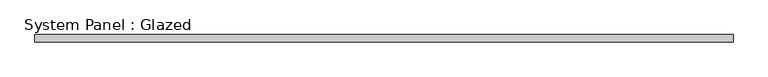
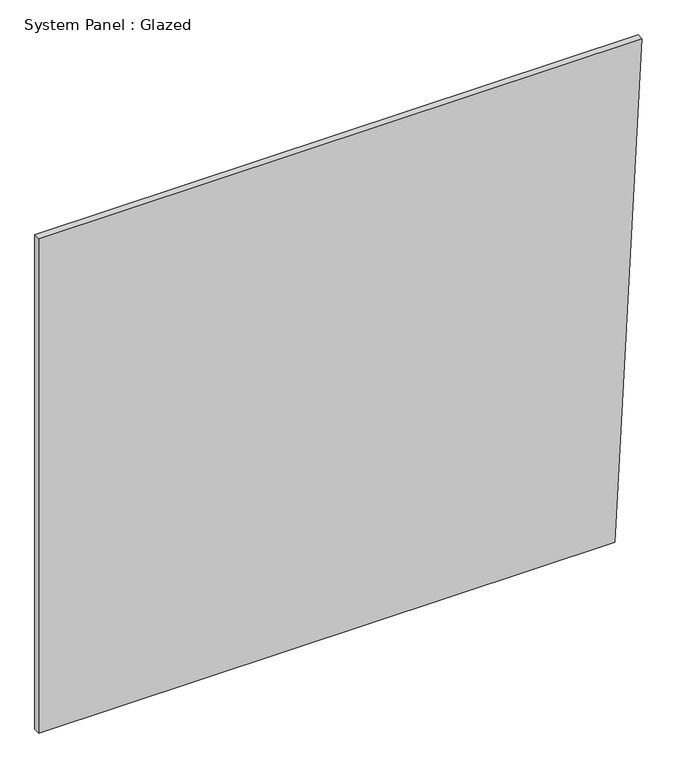
"""IFC4 building model written with IfcOpenShell, lengths in millimetres: plate geometry, System Panel : Glazed."""

import ifcopenshell
import ifcopenshell.guid

model = None  # the IFC model being written
_history = None  # IfcOwnerHistory: only IFC2X3 demands one
_inside = {}  # id of a spatial element -> (the spatial element, [elements in it])
_under = {}  # id of a project, library or spatial element -> (it, [spatial elements below it])
_declared = {}  # id of a project -> (the project, [libraries it declares])
_typed = {}  # id of a type object -> (the type object, [elements of that type])
_made_of = {}  # id of a material, layer set ... -> (it, [elements and type objects made of it])


def new_model(schema):
    """Start an empty IFC model of exactly this schema.

    Asked for "IFC4X3", IfcOpenShell would pick the latest addendum, in which some entities
    have other attributes; the version numbers below select the first issue.
    IFC2X3 requires an IfcOwnerHistory on every rooted entity: one is made here for all.
    """
    global model, _history
    if schema == "IFC4X3":
        model = ifcopenshell.file(schema_version=(4, 3, 0, 0))
    else:
        model = ifcopenshell.file(schema=schema)
    _inside.clear()
    _under.clear()
    _declared.clear()
    _typed.clear()
    _made_of.clear()
    _history = None
    if model.schema == "IFC2X3":
        org = make("IfcOrganization", Name="unknown")
        user = make(
            "IfcPersonAndOrganization",
            ThePerson=make("IfcPerson", FamilyName="unknown"),
            TheOrganization=org,
        )
        app = make(
            "IfcApplication",
            ApplicationDeveloper=org,
            Version="unknown",
            ApplicationFullName="unknown",
            ApplicationIdentifier="unknown",
        )
        _history = make(
            "IfcOwnerHistory",
            OwningUser=user,
            OwningApplication=app,
            ChangeAction="ADDED",
            CreationDate=0,
        )
    return model


def make(cls, **values):
    """One entity of the class cls with the attributes given. An attribute that is None is left unset."""
    return model.create_entity(
        cls, **{name: value for name, value in values.items() if value is not None}
    )


def rooted(cls, **values):
    """An entity with a GlobalId (a new one), such as an element, a storey or a relation."""
    return make(cls, GlobalId=ifcopenshell.guid.new(), OwnerHistory=_history, **values)


def si_unit(unit_type, name, prefix=None):
    """IfcSIUnit, for example si_unit("LENGTHUNIT", "METRE", prefix="MILLI")."""
    return make("IfcSIUnit", UnitType=unit_type, Prefix=prefix, Name=name)


def assignment(units):
    """IfcUnitAssignment: the units of a project."""
    return None if units is None else make("IfcUnitAssignment", Units=units)


def point(xyz):
    """IfcCartesianPoint."""
    return None if xyz is None else make("IfcCartesianPoint", Coordinates=xyz)


def direction(xyz):
    """IfcDirection."""
    return None if xyz is None else make("IfcDirection", DirectionRatios=xyz)


def frame(location, z_axis=None, x_axis=None):
    """IfcAxis2Placement3D, a coordinate frame: its origin and axes. An axis left out is left unset."""
    return make(
        "IfcAxis2Placement3D",
        Location=point(location),
        Axis=direction(z_axis),
        RefDirection=direction(x_axis),
    )


def origin():
    """The frame at (0, 0, 0) with its axes left unset."""
    return frame((0.0, 0.0, 0.0))


def place(relative_to, where):
    """IfcLocalPlacement: puts the frame where relative to a parent placement (None: the world)."""
    return make(
        "IfcLocalPlacement", PlacementRelTo=relative_to, RelativePlacement=where
    )


def context(
    kind, dimensions, precision=None, world=None, true_north=None, identifier=None
):
    """IfcGeometricRepresentationContext, for example the 3D "Model" context."""
    return make(
        "IfcGeometricRepresentationContext",
        ContextIdentifier=identifier,
        ContextType=kind,
        CoordinateSpaceDimension=dimensions,
        Precision=precision,
        WorldCoordinateSystem=world,
        TrueNorth=true_north,
    )


def project(units=None, contexts=None):
    """IfcProject with its units and contexts."""
    return rooted(
        "IfcProject",
        Name="project",
        RepresentationContexts=contexts,
        UnitsInContext=assignment(units),
    )


def spatial(cls, under=None, at=None, **own):
    """A site, building, storey or space (cls), placed at a placement, below another one or the project."""
    s = rooted(cls, ObjectPlacement=at, **own)
    if under is not None:
        _under.setdefault(under.id(), (under, []))[1].append(s)
    return s


def polyline(points):
    """IfcPolyline through the points."""
    return make("IfcPolyline", Points=[point(p) for p in points])


def outline(outer, holes=None, kind="AREA"):
    """IfcArbitraryClosedProfileDef: a profile drawn as a closed curve; with holes, ...WithVoids."""
    if holes is None:
        return make("IfcArbitraryClosedProfileDef", ProfileType=kind, OuterCurve=outer)
    return make(
        "IfcArbitraryProfileDefWithVoids",
        ProfileType=kind,
        OuterCurve=outer,
        InnerCurves=holes,
    )


def extrude(swept, where, along, depth):
    """IfcExtrudedAreaSolid: the profile swept, set in the frame where, extruded along a direction by depth."""
    return make(
        "IfcExtrudedAreaSolid",
        SweptArea=swept,
        Position=where,
        ExtrudedDirection=direction(along),
        Depth=depth,
    )


def shape(context_of_items, identifier, shape_type, items):
    """IfcShapeRepresentation: the items that make up one representation, for example the "Body"."""
    return make(
        "IfcShapeRepresentation",
        ContextOfItems=context_of_items,
        RepresentationIdentifier=identifier,
        RepresentationType=shape_type,
        Items=items,
    )


def source(mapping_origin, context_of_items, identifier, shape_type, items):
    """IfcRepresentationMap: a shape defined once, which mapped items show again and again."""
    return make(
        "IfcRepresentationMap",
        MappingOrigin=mapping_origin,
        MappedRepresentation=shape(context_of_items, identifier, shape_type, items),
    )


def transform(
    local_origin,
    x_axis=None,
    y_axis=None,
    z_axis=None,
    scale=None,
    scale2=None,
    scale3=None,
    uniform=True,
):
    """IfcCartesianTransformationOperator3D, or its non-uniform kind. x_axis, y_axis, z_axis: its Axis1, 2, 3."""
    if uniform:
        return make(
            "IfcCartesianTransformationOperator3D",
            Axis1=direction(x_axis),
            Axis2=direction(y_axis),
            LocalOrigin=point(local_origin),
            Scale=scale,
            Axis3=direction(z_axis),
        )
    return make(
        "IfcCartesianTransformationOperator3DnonUniform",
        Axis1=direction(x_axis),
        Axis2=direction(y_axis),
        LocalOrigin=point(local_origin),
        Scale=scale,
        Axis3=direction(z_axis),
        Scale2=scale2,
        Scale3=scale3,
    )


def mapped(mapping_source, mapping_target):
    """IfcMappedItem: shows the shape of a source again, moved by a transform."""
    return make(
        "IfcMappedItem", MappingSource=mapping_source, MappingTarget=mapping_target
    )


def made_of(thing, what):
    """Note that an element or type object is made of a material, layer set ...; save() writes the relation."""
    if what is not None:
        _made_of.setdefault(what.id(), (what, []))[1].append(thing)
    return thing


def element(
    cls,
    number,
    at=None,
    inside=None,
    cuts=None,
    type_object=None,
    material=None,
    context=None,
    identifier="Body",
    shape_type=None,
    held_by="IfcProductDefinitionShape",
    body=None,
    shapes=None,
    **own,
):
    """One element of the class cls, such as IfcWall. Its Tag is "e" and its number.

    at: its placement. inside: the storey or other place that contains it. cuts: it is an
    opening in that element (IfcRelVoidsElement). A single representation is given by context,
    identifier, shape_type and body (its items); several are given by shapes. held_by: the class
    of the entity that holds the representations. save() writes the other relations.
    """
    e = rooted(cls, Tag="e%d" % number, ObjectPlacement=at, **own)
    if body is not None:
        shapes = [shape(context, identifier, shape_type, body)]
    if shapes is not None:
        e.Representation = make(held_by, Representations=shapes)
    if inside is not None:
        _inside.setdefault(inside.id(), (inside, []))[1].append(e)
    if cuts is not None:
        rooted(
            "IfcRelVoidsElement", RelatingBuildingElement=cuts, RelatedOpeningElement=e
        )
    if type_object is not None:
        _typed.setdefault(type_object.id(), (type_object, []))[1].append(e)
    return made_of(e, material)


def aggregate(whole, parts):
    """IfcRelAggregates: a whole, such as a stair, and the parts it consists of."""
    return rooted("IfcRelAggregates", RelatingObject=whole, RelatedObjects=parts)


def save(model, path):
    """Write the relations noted so far, then the file.

    IfcRelAggregates (storeys below a building ...), IfcRelContainedInSpatialStructure (elements
    in a storey), IfcRelDefinesByType, IfcRelAssociatesMaterial and IfcRelDeclares: one each for
    every whole, place, type object, material and project.
    """
    for whole, parts in _under.values():
        aggregate(whole, parts)
    for where, things in _inside.values():
        rooted(
            "IfcRelContainedInSpatialStructure",
            RelatedElements=things,
            RelatingStructure=where,
        )
    for kind, things in _typed.values():
        rooted("IfcRelDefinesByType", RelatedObjects=things, RelatingType=kind)
    for what, things in _made_of.values():
        rooted("IfcRelAssociatesMaterial", RelatedObjects=things, RelatingMaterial=what)
    for by, libraries in _declared.values():
        rooted("IfcRelDeclares", RelatingContext=by, RelatedDefinitions=libraries)
    model.write(path)


def system_panel_glazed_bfd5517e(model_context):
    return source(origin(), model_context, "Body", "SweptSolid", [
        extrude(outline(polyline([(0.0, -1204.673413), (0.0, 1095.4915598), (2086.1728929, 1204.673413), (2086.1728929, -1204.673413), (0.0, -1204.673413)])), frame((0.0, -44.45, 0.0), z_axis=(0.0, 1.0, 0.0), x_axis=(0.0, 0.0, 1.0)), (0.0, 0.0, 1.0), 25.4),
    ])


if __name__ == "__main__":
    model = new_model("IFC4")
    model_context = context("Model", 3, world=origin())
    ifc_project = project(units=[si_unit("LENGTHUNIT", "METRE", prefix="MILLI")], contexts=[model_context])
    site = spatial("IfcSite", under=ifc_project)
    building = spatial("IfcBuilding", under=site)
    placement = place(None, origin())
    system_panel_glazed_shape = system_panel_glazed_bfd5517e(model_context)
    element("IfcPlate", 1, ObjectType="System Panel : Glazed", at=placement, inside=building, context=model_context, shape_type="MappedRepresentation", body=[
        mapped(system_panel_glazed_shape, transform((0.0, 0.0, 0.0), x_axis=(1.0, 0.0, 0.0), y_axis=(0.0, 1.0, 0.0), z_axis=(0.0, 0.0, 1.0))),
    ])
    save(model, "model.ifc")

# Revit data of these elements
# Type "System Panel : Glazed"
#   Construction Type Id = "GSP4R"
#   Analytic Construction = "1/8 in Pilkington single glazing"
#   Visual Light Transmittance = 0.9
#   Solar Heat Gain Coefficient = 0.86
#   Heat Transfer Coefficient (U) = 1.18115 BTU/(h·ft²·°F)
#   Define Thermal Properties by = 1
# Element 1 (IfcPlate, "System Panel : Glazed")
#   Materials on its faces: "Glass"
# Materials
#   "Glass": class "Glass", colour RGB 0 128 192, transparency 0.75, Description = "Soda Lime Glass", Cost = 0
